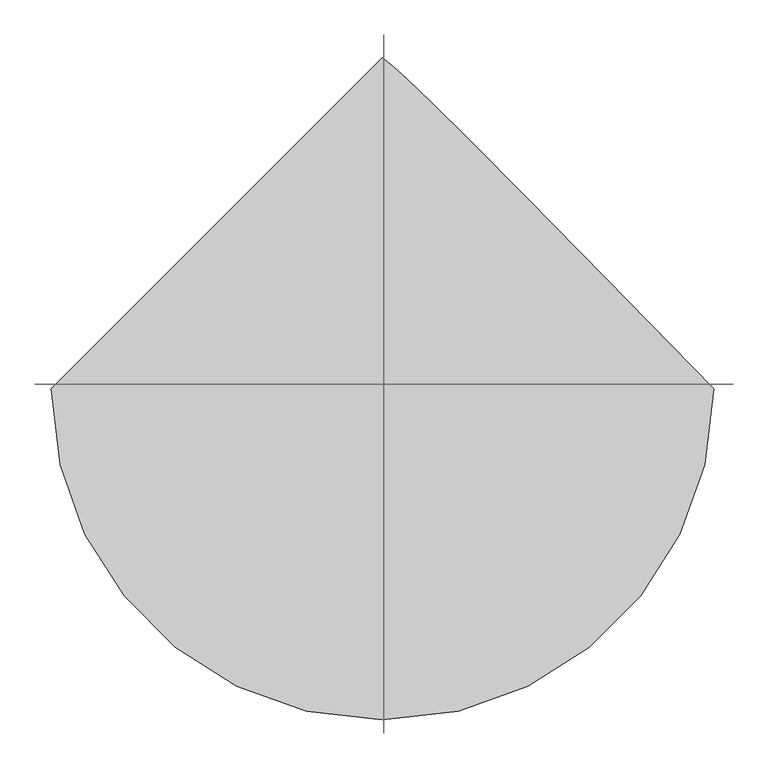
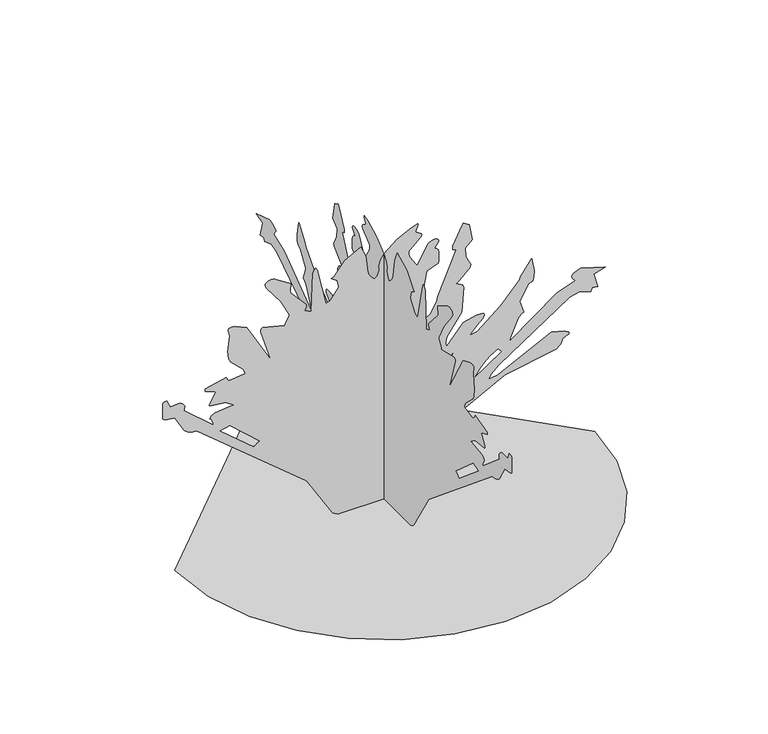
"""IFC4 building model written with IfcOpenShell, lengths in millimetres: proxy geometry, prairie dropseed 26760 : prairie dropseed 26760."""

from ifc_helpers import new_model, si_unit, origin, place, context, project, spatial, triangles, source, transform, mapped, element, save


def entourage_02fa341a(model_context):
    return source(origin(), model_context, "Body", "Tessellation", [
        triangles([(-1145.8724991, 0.0, 0.0001203), (-1115.5778366, -262.5577928, 0.0001203), (-1029.3040329, -503.6753972, 0.0001203), (-893.9573524, -716.4439871, 0.0001203), (-716.4439871, -893.9573524, 0.0001203), (-503.6753972, -1029.3040329, 0.0001203), (-262.5577928, -1115.5778366, 0.0001203), (5.01e-05, -1145.8724991, 0.0001203), (262.5577928, -1115.5778366, 0.0001203), (503.6753972, -1029.3040329, 0.0001203), (716.4439871, -893.9573524, 0.0001203), (893.9573524, -716.4439871, 0.0001203), (1029.3040329, -503.6753972, 0.0001203), (1115.5778366, -262.5577928, 0.0001203), (1145.8724991, 0.0001002, 0.0001203), (773.4874529, 381.9735961, 0.0001203), (497.4218908, 663.2029781, 0.0001203), (301.6205247, 860.4800354, 0.0001203), (170.0304827, 990.5943317, 0.0001203), (86.5989292, 1070.3377928, 0.0001203), (35.272797, 1116.4998734, 0.0001203), (-0.0001503, 1145.8724991, 0.0001203), (191.5793673, 16.4808481, 1518.7299728), (190.2057411, 16.4808481, 1512.532386), (177.5557501, 16.4808481, 1485.8293648), (178.0462362, 16.4808481, 1480.5131195), (207.8564987, 16.4808481, 1461.7196445), (211.32233, 16.4808481, 1451.7881287), (204.1071818, 16.4808481, 1439.5808796), (144.6111222, 16.4808481, 1389.2583698), (141.1229358, 16.4808481, 1381.6383408), (140.426721, 16.4808481, 1366.2256187), (146.0929631, 16.4808481, 1347.6911396), (178.4658327, 16.4808481, 1296.2230602), (186.7823127, 16.4808481, 1288.0619305), (190.0609643, 16.4808481, 1288.211776), (245.3213086, 16.4808481, 1386.9849621), (252.3454438, 16.4808481, 1394.9860725), (265.8470906, 16.4808481, 1400.4698948), (281.8237317, 16.4808481, 1402.5959278), (289.4335869, 16.4808481, 1401.7577522), (296.0960073, 16.4808481, 1399.3065937), (301.2827002, 16.4808481, 1394.9860725), (303.525532, 16.4808481, 1388.0517574), (301.6992627, 16.4808481, 1380.2565937), (279.0398718, 16.4808481, 1350.4953289), (292.1132926, 16.4808481, 1346.2916611), (300.5334, 16.4808481, 1335.2070179), (305.1155694, 16.4808481, 1319.5453285), (303.9395511, 16.4808481, 1268.0670753), (301.2827002, 16.4808481, 1257.0687641), (238.9982207, 16.4808481, 1234.823465), (219.7373687, 16.4808742, 1135.2349216), (208.8420127, 16.4808742, 1067.5641249), (212.3832936, 16.4808742, 1036.2585503), (225.652015, 16.4808742, 1007.9299015), (234.5499094, 16.4808742, 967.8917931), (248.2595922, 16.4808742, 970.7670536), (258.6512544, 16.4808742, 978.4505962), (292.3850601, 16.4808742, 1039.0729134), (298.2194605, 16.4808742, 1065.3949986), (399.1592477, 16.4808481, 1301.557037), (381.5697327, 16.4808481, 1309.1974136), (379.2862601, 16.4808481, 1328.9001354), (432.7863739, 16.4808481, 1431.8338234), (439.1998996, 16.4808481, 1439.4742001), (469.1567193, 16.4808481, 1422.9108215), (470.340368, 16.4808481, 1421.67892), (488.1381915, 16.4808481, 1328.2525005), (448.0975396, 16.4808481, 1292.6593243), (452.5450879, 16.4808481, 1243.7211777), (475.4661089, 16.4808742, 1195.1663652), (479.2405515, 16.4808742, 1190.3352648), (474.884422, 16.4808742, 1175.0165051), (415.7048584, 16.4808742, 1116.6548058), (399.1592477, 16.4808742, 1105.8064854), (400.510546, 16.4808742, 1104.4069342), (434.7498078, 16.4808742, 1083.5611135), (441.3436641, 16.4808742, 1069.7841202), (428.4937943, 16.4808742, 930.2133516), (347.4472878, 16.4808992, 815.783563), (341.366518, 16.4808992, 788.9789492), (345.7734438, 16.4808992, 758.7935097), (439.1998996, 16.4808742, 865.5651175), (512.8727283, 16.4808742, 883.5687424), (542.821954, 16.4808742, 883.172473), (547.2034452, 16.4808742, 881.851696), (550.2463918, 16.4808742, 879.4843987), (551.976119, 16.4808742, 876.1493551), (552.4231484, 16.4808742, 871.9304266), (551.610371, 16.4808742, 866.9087854), (549.5681992, 16.4808742, 861.1709089), (543.2842441, 16.4808742, 853.7287033), (531.917714, 16.4808742, 842.4993742), (517.6733437, 16.4808992, 828.930653), (502.7584474, 16.4808992, 814.4704165), (489.3751436, 16.4808992, 800.5638525), (479.7282034, 16.4808992, 788.6613813), (476.0198178, 16.4808992, 780.210807), (513.8201632, 16.4808992, 789.5783312), (642.9667133, 16.4808742, 892.3291815), (746.172187, 16.4808742, 1007.9299015), (749.7891901, 16.4808742, 1021.8363928), (808.727453, 16.4808742, 1102.2682566), (812.905759, 16.4808742, 1105.8064854), (824.3001944, 16.4808742, 1031.1582075), (823.6322119, 16.4808742, 994.8412382), (817.3558508, 16.4808742, 972.3393414), (795.110479, 16.4808742, 967.8917931), (747.0028049, 16.4808742, 882.9210348), (746.172187, 16.4808742, 878.9128492), (768.4175589, 16.4808992, 812.1793499), (753.3274189, 16.4808992, 805.8165842), (738.2855318, 16.4808992, 789.0373032), (695.1587311, 16.4808992, 686.8503719), (692.7864195, 16.4808992, 669.8145658), (947.0688635, 16.4808742, 860.4216087), (1048.699506, 16.4808742, 896.7081293), (1031.5646507, 16.4808742, 917.3609385), (1030.2641487, 16.4808742, 922.2631102), (1030.9016825, 16.4808742, 927.8511412), (1034.3306883, 16.4808742, 934.1604944), (1040.9118273, 16.4808742, 940.3403498), (1059.8323294, 16.4808742, 950.6222803), (1080.2666925, 16.4808742, 955.3314405), (1088.7376144, 16.4808742, 954.5440613), (1213.3071184, 16.4808742, 914.5034094), (1151.0236382, 16.4808742, 896.7081293), (1173.2664665, 16.4808992, 816.6268982), (1142.1259981, 16.4808992, 821.0769899), (1133.2283581, 16.4808992, 803.2817099), (1073.0276722, 16.4808742, 824.1351608), (1018.2448242, 16.4808992, 810.9525352), (631.9609171, 16.4808992, 554.5135732), (591.7932381, 16.4808992, 516.5074991), (577.1145555, 16.4808992, 491.8592943), (627.4016024, 16.4808992, 498.6258508), (914.8336218, 16.4808992, 642.3291796), (919.6799829, 16.4808992, 643.1216457), (989.570775, 16.4808992, 625.9969643), (1013.5077587, 16.4808992, 611.3792519), (1017.1018707, 16.4808992, 604.5339211), (1013.9115858, 16.4808992, 600.0584312), (1009.2633957, 16.4808992, 596.634476), (980.9245731, 16.4808992, 585.3568577), (971.1252439, 16.4808992, 556.8427915), (945.85215, 16.4808992, 537.2669515), (663.4595032, 16.4808992, 486.10365), (303.2308916, 16.4809242, 297.9146645), (169.4772643, 16.4809242, 161.3263992), (69.2098062, 16.4809242, 12.9610616), (67.9149089, 16.4809242, 9.6154435), (64.4996195, 16.4809242, 6.7499111), (47.3677937, 16.4809242, 1.1487808), (-237.5664222, 16.4809242, 3.55e-05), (-244.2689927, 16.4809242, 1.6405105), (-251.0271739, 16.4809242, 4.0836423), (-257.5565174, 16.4809242, 7.0952757), (-263.5737918, 16.4809242, 10.4413515), (-268.793495, 16.4809242, 13.8879604), (-272.9311604, 16.4809242, 17.2006602), (-275.702303, 16.4809242, 20.1455931), (-415.6845471, 16.4809242, 251.3398547), (-1015.5905531, 16.4808992, 749.8933262), (-1043.5331789, 16.4808992, 753.4493591), (-1066.7030582, 16.4808992, 763.3172161), (-1085.8064707, 16.4808992, 778.3058361), (-1135.7099653, 16.4808742, 865.5651175), (-1188.5954, 16.4808742, 874.7803253), (-1197.2085371, 16.4808742, 878.409973), (-1202.4434647, 16.4808742, 883.3603975), (-1200.9524946, 16.4808742, 970.6299253), (-1197.9959164, 16.4808742, 976.7894331), (-1180.2006363, 16.4808742, 981.2369814), (-1162.4053562, 16.4808742, 941.1963295), (-1112.0319775, 16.4808742, 943.6424011), (-1102.0192892, 16.4808742, 939.9618845), (-1092.2453945, 16.4808742, 932.1361267), (-1082.3241251, 16.4808742, 918.9535011), (-1086.0451916, 16.4808742, 894.3433754), (-1086.7716734, 16.4808742, 892.2580376), (-926.6116093, 16.4808992, 754.3434179), (-925.605784, 16.4808992, 759.362443), (-927.0764791, 16.4808992, 766.1722017), (-938.5826809, 16.4808992, 788.0010292), (-942.1971405, 16.4808992, 792.6314152), (-944.4068893, 16.4808992, 794.3840698), (-937.4142929, 16.4808992, 808.8823854), (-919.3421402, 16.4808992, 818.6817146), (-823.4569319, 16.4808742, 829.6215265), (-815.3899097, 16.4808742, 829.97463), (-858.7680759, 16.4808742, 860.6984814), (-944.4068893, 16.4808742, 870.0152092), (-947.1628258, 16.4808742, 873.2892826), (-945.4203449, 16.4808742, 881.8338919), (-918.6309191, 16.4808742, 930.5131153), (-913.2664209, 16.4808742, 936.7487812), (-916.3169615, 16.4808742, 939.0652822), (-971.1023529, 16.4808742, 963.4417013), (-971.1023529, 16.4808742, 976.7894331), (-855.4305616, 16.4808742, 1003.4823532), (-846.5329216, 16.4808742, 985.6870731), (-841.8745577, 16.4808742, 979.8552343), (-829.7383799, 16.4808742, 977.9705383), (-753.1064295, 16.4808742, 990.1346214), (-756.4770086, 16.4808742, 1006.0553793), (-765.4127277, 16.4808742, 1020.5536949), (-831.3791954, 16.4808742, 1083.2842409), (-840.7899582, 16.4808742, 1103.5102592), (-847.4701464, 16.4808742, 1148.4429817), (-835.9664881, 16.4808481, 1236.4922585), (-844.9453732, 16.4808481, 1268.2270947), (-844.5237419, 16.4808481, 1274.356081), (-842.0828299, 16.4808481, 1279.3142086), (-823.4467581, 16.4808481, 1281.6536007), (-807.3482494, 16.4808481, 1280.2336292), (-744.2087894, 16.4808481, 1252.618745), (-611.5748068, 16.4808742, 1020.9982172), (-667.4397108, 16.4808742, 1200.5004147), (-666.7716557, 16.4808742, 1209.9873356), (-663.0404154, 16.4808742, 1217.4803375), (-655.2298456, 16.4808742, 1221.4783493), (-535.1105061, 16.4808742, 1190.3352648), (-533.8786045, 16.4808742, 1199.9263218), (-512.8651342, 16.4808481, 1239.2736294), (-511.3157375, 16.4808481, 1244.1986195), (-557.3532981, 16.4808481, 1337.1500679), (-634.6126448, 16.4808481, 1439.0804741), (-643.7160135, 16.4808481, 1457.800407), (-641.8821138, 16.4808481, 1466.1671928), (-637.6073021, 16.4808481, 1471.8948956), (-632.047249, 16.4808481, 1476.1239979), (-625.5575289, 16.4808481, 1478.9915554), (-611.2090588, 16.4808481, 1481.1760151), (-597.39395, 16.4808481, 1479.5149246), (-503.9674942, 16.4808481, 1421.67892), (-502.3393596, 16.4808481, 1414.2646923), (-507.1602862, 16.4808481, 1383.6296436), (-506.7665603, 16.4808481, 1375.9283695), (-503.9674942, 16.4808481, 1368.290609), (-419.4386421, 16.4808481, 1270.4164959), (-417.9679833, 16.4808481, 1265.4483398), (-418.4759829, 16.4808481, 1259.8959171), (-428.3362822, 16.4808481, 1239.2736294), (-392.7457583, 16.4808742, 1221.4783493), (-382.6517524, 16.4808481, 1438.78587), (-376.0604396, 16.4808481, 1454.3636982), (-366.0502948, 16.4808481, 1461.7196445), (-358.5369452, 16.4808481, 1448.6461693), (-312.6644546, 16.4808481, 1243.7211777), (-312.6644546, 16.4808481, 1239.2736294), (-297.8790925, 16.4808481, 1242.0853764), (-285.9918639, 16.4808481, 1249.6164574), (-241.4823532, 16.4808481, 1310.4546043), (-250.3804838, 16.4808481, 1350.4953289), (-281.5214609, 16.4808481, 1372.7406281), (-269.5834359, 16.4808481, 1376.9621727), (-207.497836, 16.4808481, 1449.829818), (-121.3619509, 16.4808481, 1497.3102047), (-95.2247926, 16.4808481, 1437.6657349), (-83.2026885, 16.4808481, 1344.1731857), (-76.9446311, 16.4808481, 1324.6506855), (-65.1584955, 16.4808481, 1306.0909172), (-45.7307615, 16.4808481, 1288.211776), (-41.5217161, 16.4808481, 1290.5004444), (-35.9095768, 16.4808481, 1296.6929443), (-29.9423425, 16.4808481, 1305.7657917), (-24.6679461, 16.4808481, 1316.7005894), (-21.135356, 16.4808481, 1328.4811203), (-20.392126, 16.4808481, 1340.0863712), (-23.4862072, 16.4808481, 1350.4953289), (-15.2394211, 16.4808481, 1383.2867867), (6.9086104, 16.4808481, 1415.9385727), (77.353318, 16.4808481, 1474.7548954), (156.7378711, 16.4808481, 1514.8082645), (190.0609643, 16.4808481, 1524.0030521), (314.8691892, 16.4808992, 650.9652077), (302.783844, 16.4808992, 632.2733253), (297.6250927, 16.4808992, 615.8852268), (301.2827002, 16.4808992, 603.0810302), (316.0884098, 16.4808992, 608.5598019), (394.7091559, 16.4808992, 723.2004061), (-891.0210491, 16.4808992, 705.405126), (-704.1681376, 16.4808992, 549.69519), (-701.9100632, 16.4808992, 552.6847967), (-698.0060863, 16.4808992, 556.3906388), (-693.0047928, 16.4808992, 560.4190993), (-687.457457, 16.4808992, 564.3789594), (-681.9125919, 16.4808992, 567.8816525), (-676.9164579, 16.4808992, 570.5308731), (-673.0251257, 16.4808992, 571.9380183), (-837.6352816, 16.4808992, 718.7528578), (585.3822558, 16.4808992, 625.1511583), (564.2392513, 16.4808992, 606.7843652), (544.2418164, 16.4808992, 586.416059), (525.5346734, 16.4808992, 565.0190366), (508.2651607, 16.4808992, 543.5585369), (492.5857398, 16.4808992, 522.9997627), (648.2982193, 16.4808992, 625.3263657), (630.5029392, 16.4808992, 647.569194), (630.5029392, 16.4808992, 652.0192858), (5.4318519, 202.6286565, 1518.7299728), (5.4318519, 201.2550121, 1512.532386), (5.4318519, 188.6050212, 1485.8293648), (5.4318519, 189.0955072, 1480.5131195), (5.4318519, 218.9057698, 1461.7196445), (5.4318519, 222.3716011, 1451.7881287), (5.4318519, 215.156471, 1439.5808796), (5.4318519, 155.6603933, 1389.2583698), (5.4318519, 152.1722159, 1381.6383408), (5.4318519, 151.4760012, 1366.2256187), (5.4318519, 157.1419889, 1347.6911396), (5.4318519, 189.5151219, 1296.2230602), (5.4318519, 197.8316019, 1288.0619305), (5.4318519, 201.1102354, 1288.211776), (5.4318519, 256.3703253, 1386.9849621), (5.4318519, 263.3959866, 1394.9860725), (5.4318519, 276.8961073, 1400.4698948), (5.4318519, 292.8752918, 1402.5959278), (5.4318519, 300.4826036, 1401.7577522), (5.4318519, 307.145024, 1399.3065937), (5.4318519, 312.331735, 1394.9860725), (5.4318519, 314.5745487, 1388.0517574), (5.4318519, 312.7482794, 1380.2565937), (5.4318519, 290.0889067, 1350.4953289), (5.4318519, 303.1623093, 1346.2916611), (5.4318519, 311.5824348, 1335.2094887), (5.4318519, 316.1646043, 1319.5453285), (5.4318519, 314.9885859, 1268.0670753), (5.4318519, 312.331735, 1257.0687641), (5.4318519, 250.0474917, 1234.823465), (5.4318519, 230.7866398, 1135.2349216), (5.4318519, 219.8912838, 1067.5641249), (5.4318519, 223.4325647, 1036.2585503), (5.4318519, 236.7015404, 1007.9299015), (5.4318519, 245.5991804, 967.8917931), (5.4318519, 259.3091176, 970.7695971), (5.4318519, 269.7002711, 978.4531397), (5.4318519, 303.434095, 1039.0729134), (5.4318519, 309.2684772, 1065.3949986), (5.4318519, 410.2082826, 1301.557037), (5.4318519, 392.6187312, 1309.1974136), (5.4318519, 390.3378385, 1328.9001354), (5.4318519, 443.8354088, 1431.8338234), (5.4318519, 450.2489345, 1439.4742001), (5.4318519, 480.2057542, 1422.9108215), (5.4318519, 481.39191, 1421.67892), (5.4318519, 499.1871901, 1328.2525005), (5.4318519, 459.1465745, 1292.6593243), (5.4318519, 463.5941228, 1243.7236485), (5.4318519, 486.5151074, 1195.1663652), (5.4318519, 490.28955, 1190.3352648), (5.4318519, 485.9334569, 1175.0165051), (5.4318519, 426.7538569, 1116.6548058), (5.4318519, 410.2082826, 1105.8064854), (5.4318519, 411.5595809, 1104.4069342), (5.4318519, 445.7988427, 1083.5611135), (5.4318519, 452.392699, 1069.7841202), (5.4318519, 439.5427929, 930.2133516), (5.4318519, 358.4963227, 815.783563), (5.4318519, 352.4155529, 788.9789492), (5.4318519, 356.8224423, 758.7935097), (5.4318519, 450.2489345, 865.5651175), (5.4318519, 523.9217631, 883.5687424), (5.4318519, 553.8709525, 883.172473), (5.4318519, 558.2524801, 881.8542395), (5.4318519, 561.2953903, 879.4843987), (5.4318519, 563.0251539, 876.1493551), (5.4318519, 563.4721833, 871.9304266), (5.4318519, 562.6593696, 866.9087854), (5.4318519, 560.617234, 861.1709089), (5.4318519, 554.3332426, 853.7287033), (5.4318519, 542.9667126, 842.4993742), (5.4318519, 528.7223785, 828.930653), (5.4318519, 513.8074822, 814.4704165), (5.4318519, 500.4241785, 800.5638525), (5.4318519, 490.7772383, 788.6613813), (5.4318519, 487.0688164, 780.210807), (5.4318519, 524.869198, 789.5783312), (5.4318519, 654.0157482, 892.3291815), (5.4318519, 757.2237654, 1007.9299015), (5.4318519, 760.838225, 1021.8363928), (5.4318519, 819.7790314, 1102.2682566), (5.4318519, 823.9547939, 1105.8064854), (5.4318519, 835.3517727, 1031.1582075), (5.4318519, 834.6812468, 994.8412382), (5.4318519, 828.4048857, 972.3393414), (5.4318519, 806.1595139, 967.8917931), (5.4318519, 758.0518398, 882.9210348), (5.4318519, 757.2237654, 878.9128492), (5.4318519, 779.4665937, 812.1793499), (5.4318519, 764.3764538, 805.8191277), (5.4318519, 749.334494, 789.0373032), (5.4318519, 706.207766, 686.8503719), (5.4318519, 703.8353817, 669.8145658), (5.4318519, 958.1178257, 860.4216087), (5.4318519, 1059.7485409, 896.7081293), (5.4318519, 1042.6162291, 917.3609385), (5.4318519, 1041.3131836, 922.2631102), (5.4318519, 1041.9532608, 927.8511412), (5.4318519, 1045.3797232, 934.1604944), (5.4318519, 1051.9608622, 940.3403498), (5.4318519, 1070.8813643, 950.6222803), (5.4318519, 1091.3157274, 955.3314405), (5.4318519, 1099.7866493, 954.5440613), (5.4318519, 1224.3560806, 914.5034094), (5.4318519, 1162.072673, 896.7081293), (5.4318519, 1184.3155014, 816.6268982), (5.4318519, 1153.175033, 821.0769899), (5.4318519, 1144.277393, 803.2817099), (5.4318519, 1084.0767071, 824.1351608), (5.4318519, 1029.2938591, 810.9525352), (5.4318519, 643.0098793, 554.5135732), (5.4318519, 602.8422729, 516.5074991), (5.4318519, 588.1635904, 491.8592943), (5.4318519, 638.4505646, 498.6258508), (5.4318519, 925.8826567, 642.3291796), (5.4318519, 930.7289452, 643.1216457), (5.4318519, 1000.6197372, 625.9969643), (5.4318519, 1024.5567936, 611.3792519), (5.4318519, 1028.1509056, 604.5339211), (5.4318519, 1024.9606207, 600.0584312), (5.4318519, 1020.314974, 596.634476), (5.4318519, 991.9761515, 585.3568577), (5.4318519, 982.1742788, 556.8427915), (5.4318519, 956.9011848, 537.2669515), (5.4318519, 674.5085381, 486.10365), (5.4318519, 314.2799083, 297.9146645), (5.4318519, 180.5265354, 161.3261448), (5.4318519, 80.2590818, 12.9610366), (5.4318519, 78.9641845, 9.6153924), (5.4318519, 75.5488951, 6.7498855), (5.4318519, 58.4170693, 1.1487452), (5.4318519, -226.5171511, 0.0), (5.4318519, -233.2197035, 1.640475), (5.4318519, -239.9779029, 4.0835915), (5.4318519, -246.5075007, 7.0952502), (5.4318519, -252.5237577, 10.4413253), (5.4318519, -257.7419349, 13.8879093), (5.4318519, -261.8821436, 17.2006352), (5.4318519, -264.6532863, 20.1455681), (5.4318519, -404.6355123, 251.3398547), (5.4318519, -1004.5415182, 749.8933262), (5.4318519, -1032.484144, 753.4493591), (5.4318519, -1055.6540234, 763.3172161), (5.4318519, -1074.7574358, 778.3058361), (5.4318519, -1124.6609304, 865.5651175), (5.4318519, -1177.5463652, 874.7803253), (5.4318519, -1186.1595022, 878.409973), (5.4318519, -1191.3944298, 883.3603975), (5.4318519, -1189.9034597, 970.6299253), (5.4318519, -1186.9468815, 976.7894331), (5.4318519, -1169.1516741, 981.2369814), (5.4318519, -1151.356394, 941.1963295), (5.4318519, -1100.9830153, 943.6424011), (5.4318519, -1090.9702543, 939.9618845), (5.4318519, -1081.1963596, 932.1361267), (5.4318519, -1071.2750902, 918.9535011), (5.4318519, -1074.9961567, 894.3433754), (5.4318519, -1075.7226385, 892.260581), (5.4318519, -915.5626471, 754.3434179), (5.4318519, -914.5567492, 759.362443), (5.4318519, -916.0274443, 766.1722017), (5.4318519, -927.533646, 788.0010292), (5.4318519, -931.1481056, 792.6314152), (5.4318519, -933.3578545, 794.3840698), (5.4318519, -926.365258, 808.8823854), (5.4318519, -908.2905619, 818.6817146), (5.4318519, -812.407897, 829.62407), (5.4318519, -804.3408749, 829.97463), (5.4318519, -847.7165703, 860.6984814), (5.4318519, -933.3578545, 870.0152092), (5.4318519, -936.1137909, 873.2892826), (5.4318519, -934.3713827, 881.8338919), (5.4318519, -907.5818842, 930.5131153), (5.4318519, -902.2174587, 936.7487812), (5.4318519, -905.2679993, 939.0652822), (5.4318519, -960.053318, 963.4417013), (5.4318519, -960.053318, 976.7894331), (5.4318519, -844.3815268, 1003.4823532), (5.4318519, -835.4838867, 985.6870731), (5.4318519, -830.8255228, 979.8552343), (5.4318519, -818.6868015, 977.9705383), (5.4318519, -742.0573946, 990.1346214), (5.4318519, -745.4279737, 1006.0553793), (5.4318519, -754.3636929, 1020.5536949), (5.4318519, -820.3302332, 1083.2842409), (5.4318519, -829.7409233, 1103.5102592), (5.4318519, -836.4211115, 1148.4429817), (5.4318519, -824.9174532, 1236.4922585), (5.4318519, -833.8963383, 1268.2270947), (5.4318519, -833.474707, 1274.356081), (5.4318519, -831.033795, 1279.3142086), (5.4318519, -812.3977959, 1281.6536007), (5.4318519, -796.2992146, 1280.2336292), (5.4318519, -733.1597546, 1252.6212158), (5.4318519, -600.5257719, 1020.9982172), (5.4318519, -656.3906759, 1200.5004147), (5.4318519, -655.7226208, 1209.9873356), (5.4318519, -651.9913805, 1217.4803375), (5.4318519, -644.1808834, 1221.4783493), (5.4318519, -524.0614712, 1190.3352648), (5.4318519, -522.8270262, 1199.9263218), (5.4318519, -501.8160994, 1239.2736294), (5.4318519, -500.2667027, 1244.1986195), (5.4318519, -546.3042995, 1337.1500679), (5.4318519, -623.5636099, 1439.0804741), (5.4318519, -632.6669786, 1457.800407), (5.4318519, -630.8331516, 1466.1671928), (5.4318519, -626.5582672, 1471.8948956), (5.4318519, -620.9982141, 1476.1239979), (5.4318519, -614.508494, 1478.9915554), (5.4318519, -600.1600239, 1481.1760151), (5.4318519, -586.3449151, 1479.5149246), (5.4318519, -492.9184593, 1421.67892), (5.4318519, -491.2903247, 1414.2646923), (5.4318519, -496.1087079, 1383.6296436), (5.4318519, -495.7175617, 1375.9283695), (5.4318519, -492.9184593, 1368.290609), (5.4318519, -408.3896436, 1270.4164959), (5.4318519, -406.9189848, 1265.4483398), (5.4318519, -407.4269843, 1259.8959171), (5.4318519, -417.2872836, 1239.2736294), (5.4318519, -381.6967235, 1221.4783493), (5.4318519, -371.6027538, 1438.78587), (5.4318519, -365.011441, 1454.3636982), (5.4318519, -355.0012599, 1461.7196445), (5.4318519, -347.4854033, 1448.6487854), (5.4318519, -301.6154378, 1243.7236485), (5.4318519, -301.6154378, 1239.2736294), (5.4318519, -286.8300758, 1242.0853764), (5.4318519, -274.9428472, 1249.6164574), (5.4318519, -230.433064, 1310.4546043), (5.4318519, -239.3312127, 1350.4953289), (5.4318519, -270.4724442, 1372.7406281), (5.4318519, -258.5318758, 1376.9621727), (5.4318519, -196.448565, 1449.829818), (5.4318519, -110.3126707, 1497.3102047), (5.4318519, -84.1755125, 1437.6657349), (5.4318519, -72.1534174, 1344.1731857), (5.4318519, -65.895351, 1324.6506855), (5.4318519, -54.1092199, 1306.0909172), (5.4318519, -34.6814836, 1288.211776), (5.4318519, -30.4726948, 1290.5004444), (5.4318519, -24.860274, 1296.6929443), (5.4318519, -18.8929897, 1305.7657917), (5.4318519, -13.6186943, 1316.7005894), (5.4318519, -10.0861065, 1328.4811203), (5.4318519, -9.3428754, 1340.0863712), (5.4318519, -12.4369316, 1350.4953289), (5.4318519, -4.1901702, 1383.2867867), (5.4318519, 17.957861, 1415.9385727), (5.4318519, 88.4025891, 1474.7548954), (5.4318519, 167.7871422, 1514.8082645), (5.4318519, 201.1102354, 1524.0030521), (5.4318519, 325.918224, 650.9652077), (5.4318519, 313.8328789, 632.2733253), (5.4318519, 308.6741095, 615.8852268), (5.4318519, 312.331735, 603.0810302), (5.4318519, 327.1374084, 608.5598019), (5.4318519, 405.7581908, 723.2004061), (5.4318519, -879.9720869, 705.405126), (5.4318519, -693.1191027, 549.69519), (5.4318519, -690.8610283, 552.6847967), (5.4318519, -686.9570515, 556.3906388), (5.4318519, -681.9558306, 560.4190993), (5.4318519, -676.4084221, 564.3789594), (5.4318519, -670.8610863, 567.8816525), (5.4318519, -665.8674231, 570.5308731), (5.4318519, -661.9760908, 571.9380183), (5.4318519, -826.5862467, 718.7528578), (5.4318519, 596.4312907, 625.1511583), (5.4318519, 575.2882862, 606.7843652), (5.4318519, 555.290815, 586.416059), (5.4318519, 536.5837083, 565.0190366), (5.4318519, 519.3141955, 543.5585369), (5.4318519, 503.6347383, 522.9997627), (5.4318519, 659.3472542, 625.3263657), (5.4318519, 641.5519741, 647.569194), (5.4318519, 641.5519741, 652.0192858)], [[21, 22, 1], [20, 21, 1], [19, 20, 1], [18, 19, 1], [17, 18, 1], [17, 1, 2], [17, 2, 3], [17, 3, 4], [16, 17, 4], [16, 4, 5], [16, 5, 6], [16, 6, 7], [16, 7, 8], [16, 8, 9], [16, 9, 10], [16, 10, 11], [16, 11, 12], [15, 16, 12], [14, 15, 12], [13, 14, 12], [126, 127, 128], [104, 105, 106], [298, 284, 285], [298, 285, 286], [298, 286, 287], [298, 287, 288], [298, 288, 289], [298, 289, 290], [298, 290, 291], [255, 256, 257], [103, 104, 106], [128, 129, 130], [258, 259, 260], [247, 248, 249], [275, 276, 23], [275, 23, 24], [111, 112, 113], [246, 247, 249], [130, 131, 132], [128, 130, 132], [126, 128, 132], [125, 126, 132], [124, 125, 132], [123, 124, 132], [245, 246, 249], [245, 249, 250], [245, 250, 251], [173, 174, 175], [172, 173, 175], [291, 26, 27], [186, 187, 188], [199, 200, 201], [198, 199, 201], [198, 201, 202], [197, 198, 202], [197, 202, 203], [65, 66, 67], [275, 24, 25], [275, 25, 26], [103, 106, 107], [102, 103, 107], [102, 107, 108], [102, 108, 109], [102, 109, 110], [101, 102, 110], [101, 110, 111], [101, 111, 113], [101, 113, 114], [101, 114, 115], [100, 101, 115], [100, 115, 116], [141, 142, 143], [62, 63, 64], [68, 69, 70], [50, 51, 52], [213, 214, 215], [212, 213, 215], [212, 215, 216], [211, 212, 216], [141, 143, 144], [140, 141, 144], [139, 140, 144], [139, 144, 145], [297, 298, 291], [185, 186, 188], [185, 188, 189], [184, 185, 189], [258, 260, 261], [257, 258, 261], [255, 257, 261], [254, 255, 261], [254, 261, 262], [254, 262, 263], [184, 189, 190], [183, 184, 190], [211, 216, 217], [210, 211, 217], [209, 210, 217], [208, 209, 217], [207, 208, 217], [207, 217, 218], [206, 207, 218], [205, 206, 218], [72, 73, 74], [67, 68, 70], [65, 67, 70], [64, 65, 70], [62, 64, 70], [62, 70, 71], [62, 71, 72], [62, 72, 74], [62, 74, 75], [62, 75, 76], [61, 62, 76], [61, 76, 77], [60, 61, 77], [296, 297, 291], [193, 194, 195], [192, 193, 195], [192, 195, 196], [192, 196, 197], [192, 197, 203], [192, 203, 204], [191, 192, 204], [191, 204, 205], [191, 205, 218], [139, 145, 146], [139, 146, 147], [138, 139, 147], [138, 147, 148], [137, 138, 148], [136, 137, 148], [136, 148, 149], [49, 50, 52], [48, 49, 52], [47, 48, 52], [46, 47, 52], [27, 28, 29], [254, 263, 264], [295, 296, 291], [99, 100, 116], [170, 171, 172], [170, 172, 175], [169, 170, 175], [168, 169, 175], [168, 175, 176], [168, 176, 177], [168, 177, 178], [168, 178, 179], [168, 179, 180], [168, 180, 181], [168, 181, 182], [167, 168, 182], [166, 167, 182], [165, 166, 182], [164, 165, 182], [60, 77, 78], [60, 78, 79], [60, 79, 80], [59, 60, 80], [58, 59, 80], [58, 80, 81], [57, 58, 81], [57, 81, 82], [235, 236, 237], [235, 237, 238], [274, 275, 26], [294, 295, 291], [253, 254, 264], [235, 238, 239], [182, 183, 190], [299, 300, 301], [228, 229, 230], [228, 230, 231], [228, 231, 232], [228, 232, 233], [228, 233, 234], [228, 234, 235], [228, 235, 239], [227, 228, 239], [227, 239, 240], [227, 240, 241], [226, 227, 241], [226, 241, 242], [226, 242, 243], [226, 243, 244], [225, 226, 244], [224, 225, 244], [223, 224, 244], [220, 221, 222], [219, 220, 222], [218, 219, 222], [218, 222, 223], [218, 223, 244], [218, 244, 245], [282, 83, 84], [282, 84, 85], [282, 85, 86], [282, 86, 87], [282, 87, 88], [282, 88, 89], [282, 89, 90], [282, 90, 91], [282, 91, 92], [282, 92, 93], [282, 93, 94], [282, 94, 95], [282, 95, 96], [282, 96, 97], [282, 97, 98], [282, 98, 99], [282, 99, 116], [281, 282, 116], [182, 190, 191], [42, 43, 44], [42, 44, 45], [41, 42, 45], [40, 41, 45], [39, 40, 45], [38, 39, 45], [37, 38, 45], [37, 45, 46], [37, 46, 52], [36, 37, 52], [35, 36, 52], [35, 52, 53], [34, 35, 53], [83, 282, 277], [270, 271, 272], [273, 274, 26], [272, 273, 26], [270, 272, 26], [269, 270, 26], [268, 269, 26], [218, 245, 251], [151, 152, 153], [218, 251, 252], [267, 268, 26], [82, 83, 277], [57, 82, 277], [57, 277, 278], [57, 278, 279], [151, 153, 154], [252, 253, 264], [218, 252, 264], [150, 151, 154], [150, 154, 155], [150, 155, 156], [150, 156, 157], [150, 157, 158], [150, 158, 159], [150, 159, 160], [150, 160, 161], [150, 161, 162], [150, 162, 163], [149, 150, 163], [120, 121, 122], [119, 120, 122], [119, 122, 123], [118, 119, 123], [118, 123, 132], [117, 118, 132], [117, 132, 133], [117, 133, 134], [116, 117, 134], [34, 53, 54], [136, 149, 163], [135, 136, 163], [134, 135, 163], [191, 218, 264], [266, 267, 26], [266, 26, 291], [265, 266, 291], [264, 265, 291], [191, 264, 291], [191, 291, 292], [182, 191, 292], [182, 292, 283], [164, 182, 283], [164, 283, 284], [163, 164, 284], [163, 284, 298], [134, 163, 298], [134, 298, 299], [116, 134, 299], [116, 299, 301], [281, 116, 301], [281, 301, 293], [281, 293, 294], [280, 281, 294], [280, 294, 291], [279, 280, 291], [57, 279, 291], [56, 57, 291], [55, 56, 291], [54, 55, 291], [34, 54, 291], [33, 34, 291], [32, 33, 291], [31, 32, 291], [30, 31, 291], [30, 291, 27], [30, 27, 29], [405, 406, 407], [383, 384, 385], [577, 563, 564], [577, 564, 565], [577, 565, 566], [577, 566, 567], [577, 567, 568], [577, 568, 569], [577, 569, 570], [534, 535, 536], [382, 383, 385], [407, 408, 409], [537, 538, 539], [526, 527, 528], [554, 555, 302], [554, 302, 303], [390, 391, 392], [525, 526, 528], [409, 410, 411], [407, 409, 411], [405, 407, 411], [404, 405, 411], [403, 404, 411], [402, 403, 411], [524, 525, 528], [524, 528, 529], [524, 529, 530], [452, 453, 454], [451, 452, 454], [570, 305, 306], [465, 466, 467], [478, 479, 480], [477, 478, 480], [477, 480, 481], [476, 477, 481], [476, 481, 482], [344, 345, 346], [554, 303, 304], [554, 304, 305], [382, 385, 386], [381, 382, 386], [381, 386, 387], [381, 387, 388], [381, 388, 389], [380, 381, 389], [380, 389, 390], [380, 390, 392], [380, 392, 393], [380, 393, 394], [379, 380, 394], [379, 394, 395], [420, 421, 422], [341, 342, 343], [347, 348, 349], [329, 330, 331], [492, 493, 494], [491, 492, 494], [491, 494, 495], [490, 491, 495], [420, 422, 423], [419, 420, 423], [418, 419, 423], [418, 423, 424], [576, 577, 570], [464, 465, 467], [464, 467, 468], [463, 464, 468], [537, 539, 540], [536, 537, 540], [534, 536, 540], [533, 534, 540], [533, 540, 541], [533, 541, 542], [463, 468, 469], [462, 463, 469], [490, 495, 496], [489, 490, 496], [488, 489, 496], [487, 488, 496], [486, 487, 496], [486, 496, 497], [485, 486, 497], [484, 485, 497], [351, 352, 353], [346, 347, 349], [344, 346, 349], [343, 344, 349], [341, 343, 349], [341, 349, 350], [341, 350, 351], [341, 351, 353], [341, 353, 354], [341, 354, 355], [340, 341, 355], [340, 355, 356], [339, 340, 356], [575, 576, 570], [472, 473, 474], [471, 472, 474], [471, 474, 475], [471, 475, 476], [471, 476, 482], [471, 482, 483], [470, 471, 483], [470, 483, 484], [470, 484, 497], [418, 424, 425], [418, 425, 426], [417, 418, 426], [417, 426, 427], [416, 417, 427], [415, 416, 427], [415, 427, 428], [328, 329, 331], [327, 328, 331], [326, 327, 331], [325, 326, 331], [306, 307, 308], [533, 542, 543], [574, 575, 570], [378, 379, 395], [449, 450, 451], [449, 451, 454], [448, 449, 454], [447, 448, 454], [447, 454, 455], [447, 455, 456], [447, 456, 457], [447, 457, 458], [447, 458, 459], [447, 459, 460], [447, 460, 461], [446, 447, 461], [445, 446, 461], [444, 445, 461], [443, 444, 461], [339, 356, 357], [339, 357, 358], [339, 358, 359], [338, 339, 359], [337, 338, 359], [337, 359, 360], [336, 337, 360], [336, 360, 361], [514, 515, 516], [514, 516, 517], [553, 554, 305], [573, 574, 570], [532, 533, 543], [514, 517, 518], [461, 462, 469], [578, 579, 580], [507, 508, 509], [507, 509, 510], [507, 510, 511], [507, 511, 512], [507, 512, 513], [507, 513, 514], [507, 514, 518], [506, 507, 518], [506, 518, 519], [506, 519, 520], [505, 506, 520], [505, 520, 521], [505, 521, 522], [505, 522, 523], [504, 505, 523], [503, 504, 523], [502, 503, 523], [499, 500, 501], [498, 499, 501], [497, 498, 501], [497, 501, 502], [497, 502, 523], [497, 523, 524], [561, 362, 363], [561, 363, 364], [561, 364, 365], [561, 365, 366], [561, 366, 367], [561, 367, 368], [561, 368, 369], [561, 369, 370], [561, 370, 371], [561, 371, 372], [561, 372, 373], [561, 373, 374], [561, 374, 375], [561, 375, 376], [561, 376, 377], [561, 377, 378], [561, 378, 395], [560, 561, 395], [461, 469, 470], [321, 322, 323], [321, 323, 324], [320, 321, 324], [319, 320, 324], [318, 319, 324], [317, 318, 324], [316, 317, 324], [316, 324, 325], [316, 325, 331], [315, 316, 331], [314, 315, 331], [314, 331, 332], [313, 314, 332], [362, 561, 556], [549, 550, 551], [552, 553, 305], [551, 552, 305], [549, 551, 305], [548, 549, 305], [547, 548, 305], [497, 524, 530], [430, 431, 432], [497, 530, 531], [546, 547, 305], [361, 362, 556], [336, 361, 556], [336, 556, 557], [336, 557, 558], [430, 432, 433], [531, 532, 543], [497, 531, 543], [429, 430, 433], [429, 433, 434], [429, 434, 435], [429, 435, 436], [429, 436, 437], [429, 437, 438], [429, 438, 439], [429, 439, 440], [429, 440, 441], [429, 441, 442], [428, 429, 442], [399, 400, 401], [398, 399, 401], [398, 401, 402], [397, 398, 402], [397, 402, 411], [396, 397, 411], [396, 411, 412], [396, 412, 413], [395, 396, 413], [313, 332, 333], [415, 428, 442], [414, 415, 442], [413, 414, 442], [470, 497, 543], [545, 546, 305], [545, 305, 570], [544, 545, 570], [543, 544, 570], [470, 543, 570], [470, 570, 571], [461, 470, 571], [461, 571, 562], [443, 461, 562], [443, 562, 563], [442, 443, 563], [442, 563, 577], [413, 442, 577], [413, 577, 578], [395, 413, 578], [395, 578, 580], [560, 395, 580], [560, 580, 572], [560, 572, 573], [559, 560, 573], [559, 573, 570], [558, 559, 570], [336, 558, 570], [335, 336, 570], [334, 335, 570], [333, 334, 570], [313, 333, 570], [312, 313, 570], [311, 312, 570], [310, 311, 570], [309, 310, 570], [309, 570, 306], [309, 306, 308]], closed=False),
    ])


if __name__ == "__main__":
    model = new_model("IFC4")
    model_context = context("Model", 3, world=origin())
    ifc_project = project(units=[si_unit("LENGTHUNIT", "METRE", prefix="MILLI")], contexts=[model_context])
    site = spatial("IfcSite", under=ifc_project)
    building = spatial("IfcBuilding", under=site)
    placement = place(None, origin())
    entourage_shape = entourage_02fa341a(model_context)
    element("IfcBuildingElementProxy", 1, Name="prairie dropseed 26760 : prairie dropseed 26760", ObjectType="prairie dropseed 26760 : prairie dropseed 26760", at=placement, inside=building, context=model_context, shape_type="MappedRepresentation", body=[
        mapped(entourage_shape, transform((0.0, 0.0, 0.0), x_axis=(1.0, 0.0, 0.0), y_axis=(0.0, 1.0, 0.0), z_axis=(0.0, 0.0, 1.0))),
    ])
    save(model, "model.ifc")

# Revit data of these elements
# Type "prairie dropseed 26760 : prairie dropseed 26760"
#   built-in parameter 1005195 = "RPC-16-FVGU-WKFX-7K3N-J000-ST1L-LVER-AU"
#   Height = 0
